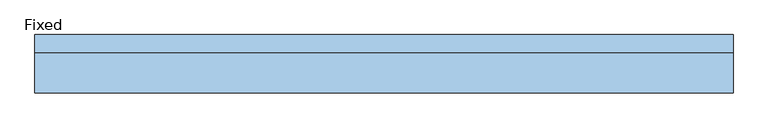
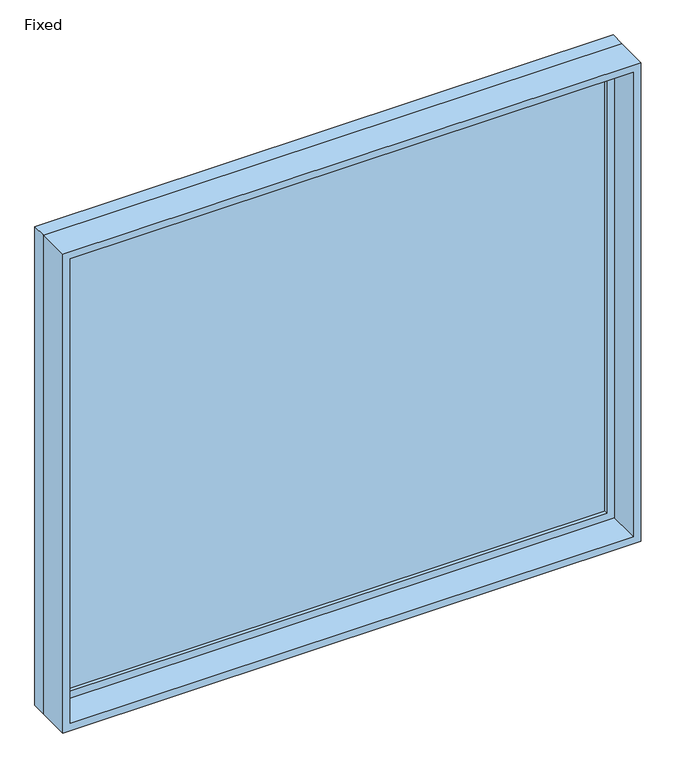
"""IFC4 building model written with IfcOpenShell, lengths in millimetres: window geometry, Fixed : dough."""

import ifcopenshell
import ifcopenshell.guid

model = None  # the IFC model being written
_history = None  # IfcOwnerHistory: only IFC2X3 demands one
_inside = {}  # id of a spatial element -> (the spatial element, [elements in it])
_under = {}  # id of a project, library or spatial element -> (it, [spatial elements below it])
_declared = {}  # id of a project -> (the project, [libraries it declares])
_typed = {}  # id of a type object -> (the type object, [elements of that type])
_made_of = {}  # id of a material, layer set ... -> (it, [elements and type objects made of it])


def new_model(schema):
    """Start an empty IFC model of exactly this schema.

    Asked for "IFC4X3", IfcOpenShell would pick the latest addendum, in which some entities
    have other attributes; the version numbers below select the first issue.
    IFC2X3 requires an IfcOwnerHistory on every rooted entity: one is made here for all.
    """
    global model, _history
    if schema == "IFC4X3":
        model = ifcopenshell.file(schema_version=(4, 3, 0, 0))
    else:
        model = ifcopenshell.file(schema=schema)
    _inside.clear()
    _under.clear()
    _declared.clear()
    _typed.clear()
    _made_of.clear()
    _history = None
    if model.schema == "IFC2X3":
        org = make("IfcOrganization", Name="unknown")
        user = make(
            "IfcPersonAndOrganization",
            ThePerson=make("IfcPerson", FamilyName="unknown"),
            TheOrganization=org,
        )
        app = make(
            "IfcApplication",
            ApplicationDeveloper=org,
            Version="unknown",
            ApplicationFullName="unknown",
            ApplicationIdentifier="unknown",
        )
        _history = make(
            "IfcOwnerHistory",
            OwningUser=user,
            OwningApplication=app,
            ChangeAction="ADDED",
            CreationDate=0,
        )
    return model


def make(cls, **values):
    """One entity of the class cls with the attributes given. An attribute that is None is left unset."""
    return model.create_entity(
        cls, **{name: value for name, value in values.items() if value is not None}
    )


def rooted(cls, **values):
    """An entity with a GlobalId (a new one), such as an element, a storey or a relation."""
    return make(cls, GlobalId=ifcopenshell.guid.new(), OwnerHistory=_history, **values)


def si_unit(unit_type, name, prefix=None):
    """IfcSIUnit, for example si_unit("LENGTHUNIT", "METRE", prefix="MILLI")."""
    return make("IfcSIUnit", UnitType=unit_type, Prefix=prefix, Name=name)


def assignment(units):
    """IfcUnitAssignment: the units of a project."""
    return None if units is None else make("IfcUnitAssignment", Units=units)


def point(xyz):
    """IfcCartesianPoint."""
    return None if xyz is None else make("IfcCartesianPoint", Coordinates=xyz)


def direction(xyz):
    """IfcDirection."""
    return None if xyz is None else make("IfcDirection", DirectionRatios=xyz)


def frame(location, z_axis=None, x_axis=None):
    """IfcAxis2Placement3D, a coordinate frame: its origin and axes. An axis left out is left unset."""
    return make(
        "IfcAxis2Placement3D",
        Location=point(location),
        Axis=direction(z_axis),
        RefDirection=direction(x_axis),
    )


def origin():
    """The frame at (0, 0, 0) with its axes left unset."""
    return frame((0.0, 0.0, 0.0))


def place(relative_to, where):
    """IfcLocalPlacement: puts the frame where relative to a parent placement (None: the world)."""
    return make(
        "IfcLocalPlacement", PlacementRelTo=relative_to, RelativePlacement=where
    )


def context(
    kind, dimensions, precision=None, world=None, true_north=None, identifier=None
):
    """IfcGeometricRepresentationContext, for example the 3D "Model" context."""
    return make(
        "IfcGeometricRepresentationContext",
        ContextIdentifier=identifier,
        ContextType=kind,
        CoordinateSpaceDimension=dimensions,
        Precision=precision,
        WorldCoordinateSystem=world,
        TrueNorth=true_north,
    )


def project(units=None, contexts=None):
    """IfcProject with its units and contexts."""
    return rooted(
        "IfcProject",
        Name="project",
        RepresentationContexts=contexts,
        UnitsInContext=assignment(units),
    )


def spatial(cls, under=None, at=None, **own):
    """A site, building, storey or space (cls), placed at a placement, below another one or the project."""
    s = rooted(cls, ObjectPlacement=at, **own)
    if under is not None:
        _under.setdefault(under.id(), (under, []))[1].append(s)
    return s


def polyline(points):
    """IfcPolyline through the points."""
    return make("IfcPolyline", Points=[point(p) for p in points])


def outline(outer, holes=None, kind="AREA"):
    """IfcArbitraryClosedProfileDef: a profile drawn as a closed curve; with holes, ...WithVoids."""
    if holes is None:
        return make("IfcArbitraryClosedProfileDef", ProfileType=kind, OuterCurve=outer)
    return make(
        "IfcArbitraryProfileDefWithVoids",
        ProfileType=kind,
        OuterCurve=outer,
        InnerCurves=holes,
    )


def extrude(swept, where, along, depth):
    """IfcExtrudedAreaSolid: the profile swept, set in the frame where, extruded along a direction by depth."""
    return make(
        "IfcExtrudedAreaSolid",
        SweptArea=swept,
        Position=where,
        ExtrudedDirection=direction(along),
        Depth=depth,
    )


def shape(context_of_items, identifier, shape_type, items):
    """IfcShapeRepresentation: the items that make up one representation, for example the "Body"."""
    return make(
        "IfcShapeRepresentation",
        ContextOfItems=context_of_items,
        RepresentationIdentifier=identifier,
        RepresentationType=shape_type,
        Items=items,
    )


def source(mapping_origin, context_of_items, identifier, shape_type, items):
    """IfcRepresentationMap: a shape defined once, which mapped items show again and again."""
    return make(
        "IfcRepresentationMap",
        MappingOrigin=mapping_origin,
        MappedRepresentation=shape(context_of_items, identifier, shape_type, items),
    )


def transform(
    local_origin,
    x_axis=None,
    y_axis=None,
    z_axis=None,
    scale=None,
    scale2=None,
    scale3=None,
    uniform=True,
):
    """IfcCartesianTransformationOperator3D, or its non-uniform kind. x_axis, y_axis, z_axis: its Axis1, 2, 3."""
    if uniform:
        return make(
            "IfcCartesianTransformationOperator3D",
            Axis1=direction(x_axis),
            Axis2=direction(y_axis),
            LocalOrigin=point(local_origin),
            Scale=scale,
            Axis3=direction(z_axis),
        )
    return make(
        "IfcCartesianTransformationOperator3DnonUniform",
        Axis1=direction(x_axis),
        Axis2=direction(y_axis),
        LocalOrigin=point(local_origin),
        Scale=scale,
        Axis3=direction(z_axis),
        Scale2=scale2,
        Scale3=scale3,
    )


def mapped(mapping_source, mapping_target):
    """IfcMappedItem: shows the shape of a source again, moved by a transform."""
    return make(
        "IfcMappedItem", MappingSource=mapping_source, MappingTarget=mapping_target
    )


def made_of(thing, what):
    """Note that an element or type object is made of a material, layer set ...; save() writes the relation."""
    if what is not None:
        _made_of.setdefault(what.id(), (what, []))[1].append(thing)
    return thing


def element(
    cls,
    number,
    at=None,
    inside=None,
    cuts=None,
    type_object=None,
    material=None,
    context=None,
    identifier="Body",
    shape_type=None,
    held_by="IfcProductDefinitionShape",
    body=None,
    shapes=None,
    **own,
):
    """One element of the class cls, such as IfcWall. Its Tag is "e" and its number.

    at: its placement. inside: the storey or other place that contains it. cuts: it is an
    opening in that element (IfcRelVoidsElement). A single representation is given by context,
    identifier, shape_type and body (its items); several are given by shapes. held_by: the class
    of the entity that holds the representations. save() writes the other relations.
    """
    e = rooted(cls, Tag="e%d" % number, ObjectPlacement=at, **own)
    if body is not None:
        shapes = [shape(context, identifier, shape_type, body)]
    if shapes is not None:
        e.Representation = make(held_by, Representations=shapes)
    if inside is not None:
        _inside.setdefault(inside.id(), (inside, []))[1].append(e)
    if cuts is not None:
        rooted(
            "IfcRelVoidsElement", RelatingBuildingElement=cuts, RelatedOpeningElement=e
        )
    if type_object is not None:
        _typed.setdefault(type_object.id(), (type_object, []))[1].append(e)
    return made_of(e, material)


def aggregate(whole, parts):
    """IfcRelAggregates: a whole, such as a stair, and the parts it consists of."""
    return rooted("IfcRelAggregates", RelatingObject=whole, RelatedObjects=parts)


def save(model, path):
    """Write the relations noted so far, then the file.

    IfcRelAggregates (storeys below a building ...), IfcRelContainedInSpatialStructure (elements
    in a storey), IfcRelDefinesByType, IfcRelAssociatesMaterial and IfcRelDeclares: one each for
    every whole, place, type object, material and project.
    """
    for whole, parts in _under.values():
        aggregate(whole, parts)
    for where, things in _inside.values():
        rooted(
            "IfcRelContainedInSpatialStructure",
            RelatedElements=things,
            RelatingStructure=where,
        )
    for kind, things in _typed.values():
        rooted("IfcRelDefinesByType", RelatedObjects=things, RelatingType=kind)
    for what, things in _made_of.values():
        rooted("IfcRelAssociatesMaterial", RelatedObjects=things, RelatingMaterial=what)
    for by, libraries in _declared.values():
        rooted("IfcRelDeclares", RelatingContext=by, RelatedDefinitions=libraries)
    model.write(path)


def fixed_de4811a9(model_context):
    return source(origin(), model_context, "Body", "SweptSolid", [
        extrude(outline(polyline([(1117.6, 53.975), (-1193.8, 53.975), (-1193.8, 66.675), (1117.6, 66.675), (1117.6, 53.975)])), frame((0.0, 0.0, 1282.7), z_axis=(0.0, 0.0, 1.0), x_axis=(1.0, 0.0, 0.0)), (0.0, 0.0, 1.0), 2006.6),
        extrude(outline(polyline([(3333.75, -1238.25), (1238.25, -1238.25), (1238.25, 1162.05), (3333.75, 1162.05), (3333.75, -1238.25)]), holes=[polyline([(3289.3, -1193.8), (3289.3, 1117.6), (1282.7, 1117.6), (1282.7, -1193.8), (3289.3, -1193.8)])]), frame((0.0, 38.1, 0.0), z_axis=(0.0, 1.0, 0.0), x_axis=(0.0, 0.0, 1.0)), (0.0, 0.0, 1.0), 44.45),
        extrude(outline(polyline([(3352.8, -1257.3), (1219.2, -1257.3), (1219.2, 1181.1), (3352.8, 1181.1), (3352.8, -1257.3)]), holes=[polyline([(3321.05, -1225.55), (3321.05, 1149.35), (1250.95, 1149.35), (1250.95, -1225.55), (3321.05, -1225.55)])]), frame((0.0, -101.6, 0.0), z_axis=(0.0, 1.0, 0.0), x_axis=(0.0, 0.0, 1.0)), (0.0, 0.0, 1.0), 139.7),
        extrude(outline(polyline([(3352.8, 1181.1), (3352.8, -1257.3), (1219.2, -1257.3), (1219.2, 1181.1), (3352.8, 1181.1)]), holes=[polyline([(3333.75, 1162.05), (1238.25, 1162.05), (1238.25, -1238.25), (3333.75, -1238.25), (3333.75, 1162.05)])]), frame((0.0, 38.1, 0.0), z_axis=(0.0, 1.0, 0.0), x_axis=(0.0, 0.0, 1.0)), (0.0, 0.0, 1.0), 63.5),
    ])


if __name__ == "__main__":
    model = new_model("IFC4")
    model_context = context("Model", 3, world=origin())
    ifc_project = project(units=[si_unit("LENGTHUNIT", "METRE", prefix="MILLI")], contexts=[model_context])
    site = spatial("IfcSite", under=ifc_project)
    building = spatial("IfcBuilding", under=site)
    placement = place(None, origin())
    fixed_shape = fixed_de4811a9(model_context)
    element("IfcWindow", 1, ObjectType="Fixed : dough", at=placement, inside=building, context=model_context, shape_type="MappedRepresentation", body=[
        mapped(fixed_shape, transform((0.0, 0.0, 0.0), x_axis=(1.0, 0.0, 0.0), y_axis=(0.0, 1.0, 0.0), z_axis=(0.0, 0.0, 1.0))),
    ])
    save(model, "model.ifc")

# Revit data of these elements
# Type "Fixed : dough"
#   Type Mark = "13"
#   Assembly Code = "B2020100"
#   Height = 7' - 0"
#   Default Sill Height = 4' - 0"
#   Width = 8' - 0"
#   Window Inset = 0' - 0 3/4"
#   Glass Pane Material = INSULATED GLAZING
#   Sash Material = Dark metal
#   Wall Closure = (empty or 0)
# Element 1 (IfcWindow, "Fixed : dough")
#   Materials on its faces: "Dark metal", "INSULATED GLAZING"
# Materials
#   "INSULATED GLAZING": class "Glass", colour RGB 236 240 239, transparency 0.42, Description = "Soda Lime Glass", Cost = 0
#   "Dark metal": class "Generic", colour RGB 44 29 29, transparency 0, Cost = 0
